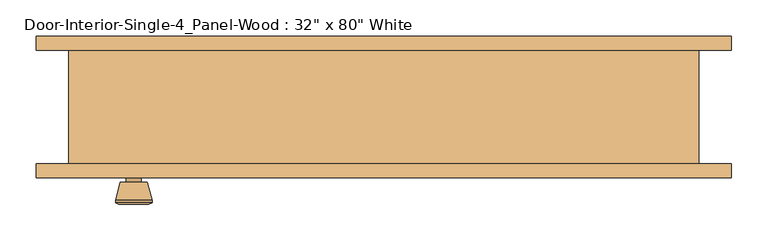
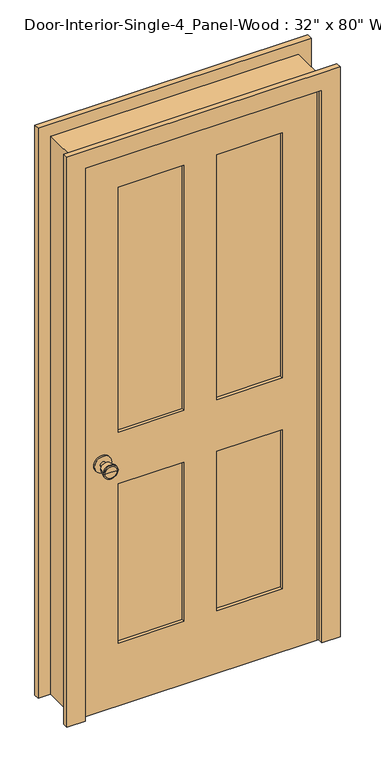
"""IFC4 building model written with IfcOpenShell, lengths in millimetres: door geometry."""

from ifc_helpers import new_model, si_unit, point, frame, frame_2d, origin, place, context, project, spatial, polyline, circle_curve, trimmed, segment, composite_curve, outline, extrude, faceted_brep, source, transform, mapped, element, save
from ifc_brep_helpers import plane_surface, cylinder_surface, revolved_surface, advanced_brep


def door_3f425913(model_context):
    return source(origin(), model_context, "Body", "SolidModel", [
        advanced_brep(
        [(-342.9, -33.6875, 914.4), (-352.9, -33.6875, 914.4), (-332.9, -33.6875, 914.4), (-322.4241324, 15.3125, 914.4), (-363.3758676, 15.3125, 914.4), (-342.9, 15.3125, 914.4), (-317.9, 13.4846319, 914.4), (-367.9, 13.4846319, 914.4), (-317.9, 10.0209537, 914.4), (-367.9, 10.0209537, 914.4), (-324.263764, -14.6875, 914.4), (-361.536236, -14.6875, 914.4), (-332.9, -14.6875, 914.4), (-352.9, -14.6875, 914.4)],
        [
            (0, 1),
            (1, 2, circle_curve(frame((-342.9, -33.6875, 914.4), z_axis=(0.0, -1.0, 0.0), x_axis=(-1.0, 0.0, 0.0)), 10.0)),
            (2, 0),
            (2, 1, circle_curve(frame((-342.9, -33.6875, 914.4), z_axis=(0.0, -1.0, 0.0), x_axis=(-1.0, 0.0, 0.0)), 10.0)),
            (3, 4, circle_curve(frame((-342.9, 15.3125, 914.4), z_axis=(0.0, 1.0, 0.0), x_axis=(-1.0, 0.0, 0.0)), 20.4758676)),
            (4, 5),
            (5, 3),
            (4, 3, circle_curve(frame((-342.9, 15.3125, 914.4), z_axis=(0.0, 1.0, 0.0), x_axis=(-1.0, 0.0, 0.0)), 20.4758676)),
            (6, 7, circle_curve(frame((-342.9, 13.4846319, 914.4), z_axis=(0.0, 1.0, 0.0), x_axis=(-1.0, 0.0, 0.0)), 25.0)),
            (7, 4),
            (3, 6),
            (7, 6, circle_curve(frame((-342.9, 13.4846319, 914.4), z_axis=(0.0, 1.0, 0.0), x_axis=(-1.0, 0.0, 0.0)), 25.0)),
            (8, 9, circle_curve(frame((-342.9, 10.0209537, 914.4), z_axis=(0.0, 1.0, 0.0), x_axis=(-1.0, 0.0, 0.0)), 25.0)),
            (9, 7),
            (6, 8),
            (9, 8, circle_curve(frame((-342.9, 10.0209537, 914.4), z_axis=(0.0, 1.0, 0.0), x_axis=(-1.0, 0.0, 0.0)), 25.0)),
            (10, 11, circle_curve(frame((-342.9, -14.6875, 914.4), z_axis=(0.0, 1.0, 0.0), x_axis=(-1.0, 0.0, 0.0)), 18.636236)),
            (11, 9),
            (8, 10),
            (11, 10, circle_curve(frame((-342.9, -14.6875, 914.4), z_axis=(0.0, 1.0, 0.0), x_axis=(-1.0, 0.0, 0.0)), 18.636236)),
            (12, 13, circle_curve(frame((-342.9, -14.6875, 914.4), z_axis=(0.0, 1.0, 0.0), x_axis=(-1.0, 0.0, 0.0)), 10.0)),
            (13, 11),
            (10, 12),
            (13, 12, circle_curve(frame((-342.9, -14.6875, 914.4), z_axis=(0.0, 1.0, 0.0), x_axis=(-1.0, 0.0, 0.0)), 10.0)),
            (1, 13),
            (12, 2),
        ],
        [
            plane_surface(frame((-342.9, -33.6875, 914.4), z_axis=(0.0, -1.0, 0.0), x_axis=(-1.0, 0.0, 0.0))),
            plane_surface(frame((-342.9, 15.3125, 914.4), z_axis=(0.0, 1.0, 0.0), x_axis=(-1.0, 0.0, 0.0))),
            revolved_surface(polyline([(-363.3758676, 15.3125, 914.4), (-367.9, 13.4846319, 914.4)]), (-342.9, -33.6875, 914.4), (0.0, -1.0, 0.0)),
            cylinder_surface(frame((-342.9, -33.6875, 914.4), z_axis=(0.0, -1.0, 0.0), x_axis=(-1.0, 0.0, 0.0)), 25.0),
            revolved_surface(polyline([(-367.9, 10.0209537, 914.4), (-361.536236, -14.6875, 914.4)]), (-342.9, -33.6875, 914.4), (0.0, -1.0, 0.0)),
            plane_surface(frame((-342.9, -14.6875, 914.4), z_axis=(0.0, -1.0, 0.0), x_axis=(-1.0, 0.0, 0.0))),
            cylinder_surface(frame((-342.9, -33.6875, 914.4), z_axis=(0.0, -1.0, 0.0), x_axis=(-1.0, 0.0, 0.0)), 10.0),
        ],
        [
            (0, [[1, 2, 3]]),
            (0, [[-3, 4, -1]]),
            (1, [[5, 6, 7]]),
            (1, [[8, -7, -6]]),
            (2, [[9, 10, -5, 11]]),
            (2, [[12, -11, -8, -10]]),
            (3, [[13, 14, -9, 15]]),
            (3, [[16, -15, -12, -14]]),
            (4, [[17, 18, -13, 19]]),
            (4, [[20, -19, -16, -18]]),
            (5, [[21, 22, -17, 23]]),
            (5, [[24, -23, -20, -22]]),
            (6, [[-2, 25, -21, 26]]),
            (6, [[-4, -26, -24, -25]]),
        ],
    ),
        extrude(outline(composite_curve([segment(trimmed(circle_curve(frame_2d((914.4, -342.9)), 30.0), [point((914.4, -372.9))], [point((914.4, -312.9))], False, "CARTESIAN"), True, "CONTINUOUS"), segment(trimmed(circle_curve(frame_2d((914.4, -342.9)), 30.0), [point((914.4, -312.9))], [point((914.4, -372.9))], False, "CARTESIAN"), True, "CONTINUOUS")], self_intersect=False)), frame((0.0, -39.6875, 0.0), z_axis=(0.0, 1.0, 0.0), x_axis=(0.0, 0.0, 1.0)), (0.0, 0.0, 1.0), 6.0),
        advanced_brep(
        [(-342.9, -80.6125, 914.4), (-332.9, -80.6125, 914.4), (-352.9, -80.6125, 914.4), (-322.4241324, -129.6125, 914.4), (-342.9, -129.6125, 914.4), (-363.3758676, -129.6125, 914.4), (-317.9, -127.7846319, 914.4), (-367.9, -127.7846319, 914.4), (-317.9, -124.3209537, 914.4), (-367.9, -124.3209537, 914.4), (-324.263764, -99.6125, 914.4), (-361.536236, -99.6125, 914.4), (-332.9, -99.6125, 914.4), (-352.9, -99.6125, 914.4)],
        [
            (0, 1),
            (1, 2, circle_curve(frame((-342.9, -80.6125, 914.4), z_axis=(0.0, 1.0, 0.0), x_axis=(-1.0, 0.0, 0.0)), 10.0)),
            (2, 0),
            (2, 1, circle_curve(frame((-342.9, -80.6125, 914.4), z_axis=(0.0, 1.0, 0.0), x_axis=(-1.0, 0.0, 0.0)), 10.0)),
            (3, 4),
            (4, 5),
            (5, 3, circle_curve(frame((-342.9, -129.6125, 914.4), z_axis=(0.0, -1.0, 0.0), x_axis=(-1.0, 0.0, 0.0)), 20.4758676)),
            (3, 5, circle_curve(frame((-342.9, -129.6125, 914.4), z_axis=(0.0, -1.0, 0.0), x_axis=(-1.0, 0.0, 0.0)), 20.4758676)),
            (6, 3),
            (5, 7),
            (7, 6, circle_curve(frame((-342.9, -127.7846319, 914.4), z_axis=(0.0, -1.0, 0.0), x_axis=(-1.0, 0.0, 0.0)), 25.0)),
            (6, 7, circle_curve(frame((-342.9, -127.7846319, 914.4), z_axis=(0.0, -1.0, 0.0), x_axis=(-1.0, 0.0, 0.0)), 25.0)),
            (8, 6),
            (7, 9),
            (9, 8, circle_curve(frame((-342.9, -124.3209537, 914.4), z_axis=(0.0, -1.0, 0.0), x_axis=(-1.0, 0.0, 0.0)), 25.0)),
            (8, 9, circle_curve(frame((-342.9, -124.3209537, 914.4), z_axis=(0.0, -1.0, 0.0), x_axis=(-1.0, 0.0, 0.0)), 25.0)),
            (10, 8),
            (9, 11),
            (11, 10, circle_curve(frame((-342.9, -99.6125, 914.4), z_axis=(0.0, -1.0, 0.0), x_axis=(-1.0, 0.0, 0.0)), 18.636236)),
            (10, 11, circle_curve(frame((-342.9, -99.6125, 914.4), z_axis=(0.0, -1.0, 0.0), x_axis=(-1.0, 0.0, 0.0)), 18.636236)),
            (12, 10),
            (11, 13),
            (13, 12, circle_curve(frame((-342.9, -99.6125, 914.4), z_axis=(0.0, -1.0, 0.0), x_axis=(-1.0, 0.0, 0.0)), 10.0)),
            (12, 13, circle_curve(frame((-342.9, -99.6125, 914.4), z_axis=(0.0, -1.0, 0.0), x_axis=(-1.0, 0.0, 0.0)), 10.0)),
            (1, 12),
            (13, 2),
        ],
        [
            plane_surface(frame((-342.9, -80.6125, 914.4), z_axis=(0.0, 1.0, 0.0), x_axis=(-1.0, 0.0, 0.0))),
            plane_surface(frame((-342.9, -129.6125, 914.4), z_axis=(0.0, -1.0, 0.0), x_axis=(-1.0, 0.0, 0.0))),
            revolved_surface(polyline([(-363.3758676, -129.6125, 914.4), (-367.9, -127.7846319, 914.4)]), (-342.9, -80.6125, 914.4), (0.0, 1.0, 0.0)),
            cylinder_surface(frame((-342.9, -80.6125, 914.4), z_axis=(0.0, 1.0, 0.0), x_axis=(-1.0, 0.0, 0.0)), 25.0),
            revolved_surface(polyline([(-367.9, -124.3209537, 914.4), (-361.536236, -99.6125, 914.4)]), (-342.9, -80.6125, 914.4), (0.0, 1.0, 0.0)),
            plane_surface(frame((-342.9, -99.6125, 914.4), z_axis=(0.0, 1.0, 0.0), x_axis=(-1.0, 0.0, 0.0))),
            cylinder_surface(frame((-342.9, -80.6125, 914.4), z_axis=(0.0, 1.0, 0.0), x_axis=(-1.0, 0.0, 0.0)), 10.0),
        ],
        [
            (0, [[1, 2, 3]]),
            (0, [[-3, 4, -1]]),
            (1, [[5, 6, 7]]),
            (1, [[-6, -5, 8]]),
            (2, [[9, -7, 10, 11]]),
            (2, [[-10, -8, -9, 12]]),
            (3, [[13, -11, 14, 15]]),
            (3, [[-14, -12, -13, 16]]),
            (4, [[17, -15, 18, 19]]),
            (4, [[-18, -16, -17, 20]]),
            (5, [[21, -19, 22, 23]]),
            (5, [[-22, -20, -21, 24]]),
            (6, [[25, -23, 26, -2]]),
            (6, [[-26, -24, -25, -4]]),
        ],
    ),
        extrude(outline(composite_curve([segment(trimmed(circle_curve(frame_2d((914.4, -342.9)), 30.0), [point((914.4, -372.9))], [point((914.4, -312.9))], False, "CARTESIAN"), True, "CONTINUOUS"), segment(trimmed(circle_curve(frame_2d((914.4, -342.9)), 30.0), [point((914.4, -312.9))], [point((914.4, -372.9))], False, "CARTESIAN"), True, "CONTINUOUS")], self_intersect=False)), frame((0.0, -80.6125, 0.0), z_axis=(0.0, 1.0, 0.0), x_axis=(0.0, 0.0, 1.0)), (0.0, 0.0, 1.0), 6.0),
        extrude(outline(polyline([(285.75, -51.3291667), (285.75, -62.9708333), (57.15, -62.9708333), (57.15, -51.3291667), (285.75, -51.3291667)])), frame((0.0, 0.0, 1009.65), z_axis=(0.0, 0.0, 1.0), x_axis=(1.0, 0.0, 0.0)), (0.0, 0.0, 1.0), 903.2875),
        extrude(outline(polyline([(-57.15, -51.3291667), (-57.15, -62.9708333), (-285.75, -62.9708333), (-285.75, -51.3291667), (-57.15, -51.3291667)])), frame((0.0, 0.0, 1009.65), z_axis=(0.0, 0.0, 1.0), x_axis=(1.0, 0.0, 0.0)), (0.0, 0.0, 1.0), 903.2875),
        extrude(outline(polyline([(285.75, -51.3291667), (285.75, -62.9708333), (57.15, -62.9708333), (57.15, -51.3291667), (285.75, -51.3291667)])), frame((0.0, 0.0, 231.775), z_axis=(0.0, 0.0, 1.0), x_axis=(1.0, 0.0, 0.0)), (0.0, 0.0, 1.0), 587.375),
        extrude(outline(polyline([(-57.15, -51.3291667), (-57.15, -62.9708333), (-285.75, -62.9708333), (-285.75, -51.3291667), (-57.15, -51.3291667)])), frame((0.0, 0.0, 231.775), z_axis=(0.0, 0.0, 1.0), x_axis=(1.0, 0.0, 0.0)), (0.0, 0.0, 1.0), 587.375),
        extrude(outline(polyline([(2032.0, -406.4), (0.0, -406.4), (0.0, 406.4), (2032.0, 406.4), (2032.0, -406.4)]), holes=[polyline([(1912.9375, 57.15), (1912.9375, 285.75), (1009.65, 285.75), (1009.65, 57.15), (1912.9375, 57.15)]), polyline([(1009.65, -57.15), (1009.65, -285.75), (1912.9375, -285.75), (1912.9375, -57.15), (1009.65, -57.15)]), polyline([(819.15, 57.15), (819.15, 285.75), (231.775, 285.75), (231.775, 57.15), (819.15, 57.15)]), polyline([(231.775, -57.15), (231.775, -285.75), (819.15, -285.75), (819.15, -57.15), (231.775, -57.15)])]), frame((0.0, -74.6125, 0.0), z_axis=(0.0, 1.0, 0.0), x_axis=(0.0, 0.0, 1.0)), (0.0, 0.0, 1.0), 34.925),
        faceted_brep([(431.8, -74.6125, 0.0), (406.4, -74.6125, 0.0), (406.4, -39.6875, 0.0), (393.7, -39.6875, 0.0), (393.7, -4.7625, 0.0), (406.4, -4.7625, 0.0), (406.4, 80.9625, 0.0), (431.8, 80.9625, 0.0), (431.8, 80.9625, 2057.4), (431.8, -74.6125, 2057.4), (406.4, 80.9625, 2032.0), (-406.4, 80.9625, 2032.0), (-406.4, 80.9625, 0.0), (-431.8, 80.9625, 0.0), (-431.8, 80.9625, 2057.4), (406.4, -4.7625, 2032.0), (393.7, -4.7625, 2019.3), (-393.7, -4.7625, 2019.3), (-393.7, -4.7625, 0.0), (-406.4, -4.7625, 0.0), (-406.4, -4.7625, 2032.0), (393.7, -39.6875, 2019.3), (406.4, -39.6875, 2032.0), (-406.4, -39.6875, 2032.0), (-406.4, -39.6875, 0.0), (-393.7, -39.6875, 0.0), (-393.7, -39.6875, 2019.3), (406.4, -74.6125, 2032.0), (-431.8, -74.6125, 2057.4), (-431.8, -74.6125, 0.0), (-406.4, -74.6125, 0.0), (-406.4, -74.6125, 2032.0)], [[[0, 1, 2, 3, 4, 5, 6, 7]], [[7, 8, 9, 0]], [[6, 10, 11, 12, 13, 14, 8, 7]], [[5, 15, 10, 6]], [[4, 16, 17, 18, 19, 20, 15, 5]], [[3, 21, 16, 4]], [[2, 22, 23, 24, 25, 26, 21, 3]], [[1, 27, 22, 2]], [[0, 9, 28, 29, 30, 31, 27, 1]], [[8, 14, 28, 9]], [[15, 20, 11, 10]], [[21, 26, 17, 16]], [[27, 31, 23, 22]], [[29, 13, 12, 19, 18, 25, 24, 30]], [[14, 13, 29, 28]], [[20, 19, 12, 11]], [[26, 25, 18, 17]], [[31, 30, 24, 23]]]),
        extrude(outline(polyline([(0.0, 476.25), (2101.85, 476.25), (2101.85, -476.25), (0.0, -476.25), (0.0, -412.75), (2038.35, -412.75), (2038.35, 412.75), (0.0, 412.75), (0.0, 476.25)])), frame((0.0, 80.9625, 0.0), z_axis=(0.0, 1.0, 0.0), x_axis=(0.0, 0.0, 1.0)), (0.0, 0.0, 1.0), 19.05),
        extrude(outline(polyline([(0.0, 476.25), (2101.85, 476.25), (2101.85, -476.25), (0.0, -476.25), (0.0, -412.75), (2038.35, -412.75), (2038.35, 412.75), (0.0, 412.75), (0.0, 476.25)])), frame((0.0, -93.6625, 0.0), z_axis=(0.0, 1.0, 0.0), x_axis=(0.0, 0.0, 1.0)), (0.0, 0.0, 1.0), 19.05),
    ])


if __name__ == "__main__":
    model = new_model("IFC4")
    model_context = context("Model", 3, world=origin())
    ifc_project = project(units=[si_unit("LENGTHUNIT", "METRE", prefix="MILLI")], contexts=[model_context])
    site = spatial("IfcSite", under=ifc_project)
    building = spatial("IfcBuilding", under=site)
    placement = place(None, origin())
    door_shape = door_3f425913(model_context)
    element("IfcDoor", 1, ObjectType="Door-Interior-Single-4_Panel-Wood : 32\" x 80\" White", at=placement, inside=building, context=model_context, shape_type="MappedRepresentation", body=[
        mapped(door_shape, transform((0.0, 0.0, 0.0), x_axis=(1.0, 0.0, 0.0), y_axis=(0.0, 1.0, 0.0), z_axis=(0.0, 0.0, 1.0))),
    ])
    save(model, "model.ifc")

# Revit data of these elements
# Type "Door-Interior-Single-4_Panel-Wood : 32\" x 80\" White"
#   Type Mark = "48"
#   COBie.Type.CreatedBy = "doug.wood@us.ibm.com"
#   COBie.Type.CreatedOn = "2016-04-14T02:07:24"
#   COBie.Type.Name = "Doors_Door-Interior-Single-4_Panel-Wood_32\" x 80\" White_48"
#   COBie.Type.Category = "23-30 10 00 : Doors"
#   COBie.Type.Description = "Door-Interior-Single-4_Panel-Wood_32\" x 80\" White"
#   COBie.Type.Manufacturer = ""
#   COBie.Type.ModelNumber = ""
#   Assembly Code = "C1020300"
#   Analytic Construction = "Wooden"
#   COBie.Type.ReplacementCost = 0
#   Top Rail = 0' - 4 11/16"
#   Thickness = 0' - 1 3/8"
#   Thermal Resistance (R) = 0.455703 (m²·K)/W
#   Swing Angle [instance default] = 90.00°
#   Stiles = 0' - 4 3/4"
#   Rough Width = 2' - 10"
#   Rough Height = 6' - 9"
#   Mullion = 0' - 4 1/2"
#   Lock Rail = 0' - 7 1/2"
#   Height = 6' - 8"
#   Width = 2' - 8"
#   Heat Transfer Coefficient (U) = 2.19465 W/(m²·K)
#   Bottom Rail = 0' - 9 1/8"
#   COBie.Type = no
#   Trim Material = Trim - White
#   Panel Material = Door - Panel - White
#   Frame Material = Door - Panel - White
#   Door Handle Material = ARCAT - Metal - Brass, Polished
#   Visual Light Transmittance = 0
#   Solar Heat Gain Coefficient = 0
#   Wall Closure = (empty or 0)
#   Function = (empty or 0)
# Element 1 (IfcDoor, "Door-Interior-Single-4_Panel-Wood : 32\" x 80\" White")
#   Materials on its faces: "Door - Panel - White", "ARCAT - Metal - Brass, Polished", "Trim - White"
# Materials
#   "Trim - White": class "Wood", colour RGB 255 255 255, transparency 0, Cost = 0
#   "Door - Panel - White": class "Wood", colour RGB 255 255 255, transparency 0, Cost = 0
#   "ARCAT - Metal - Brass, Polished": class "Unassigned", colour RGB 246 240 166, transparency 0, Keynote = "05050", Model = "Generic", Manufacturer = "Generic", Description = "Steel, Chrome Plated"
